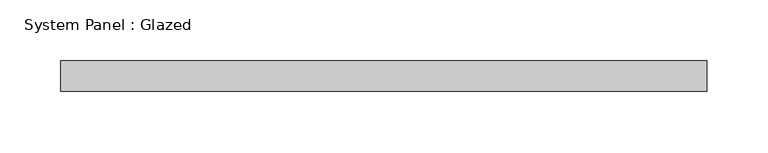
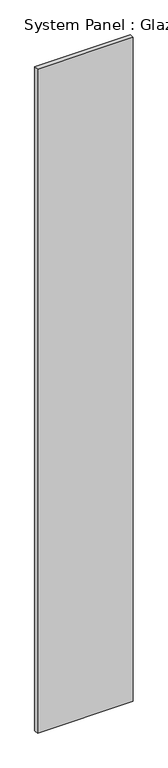
"""IFC4 building model written with IfcOpenShell, lengths in millimetres: plate geometry, System Panel : Glazed."""

from ifc_helpers import new_model, si_unit, origin, origin_with_axes, place, context, project, spatial, polyline, outline, extrude, source, transform, mapped, element, save


def system_panel_glazed_88fcc8eb(model_context):
    return source(origin(), model_context, "Body", "SweptSolid", [
        extrude(outline(polyline([(266.25, 24.5), (-266.25, 24.5), (-266.25, 49.5), (266.25, 49.5), (266.25, 24.5)])), origin_with_axes(), (0.0, 0.0, 1.0), 3900.0),
    ])


if __name__ == "__main__":
    model = new_model("IFC4")
    model_context = context("Model", 3, world=origin())
    ifc_project = project(units=[si_unit("LENGTHUNIT", "METRE", prefix="MILLI")], contexts=[model_context])
    site = spatial("IfcSite", under=ifc_project)
    building = spatial("IfcBuilding", under=site)
    placement = place(None, origin())
    system_panel_glazed_shape = system_panel_glazed_88fcc8eb(model_context)
    element("IfcPlate", 1, ObjectType="System Panel : Glazed", at=placement, inside=building, context=model_context, shape_type="MappedRepresentation", body=[
        mapped(system_panel_glazed_shape, transform((0.0, 0.0, 0.0), x_axis=(1.0, 0.0, 0.0), y_axis=(0.0, 1.0, 0.0), z_axis=(0.0, 0.0, 1.0))),
    ])
    save(model, "model.ifc")

# Revit data of these elements
# Type "System Panel : Glazed"
#   Keynote = "H11"
#   Construction Type Id = "GSP4R"
#   Analytic Construction = "1/8 in Pilkington single glazing"
#   Visual Light Transmittance = 0.9
#   Solar Heat Gain Coefficient = 0.86
#   Heat Transfer Coefficient (U) = 6.7069 W/(m²·K)
#   Define Thermal Properties by = 1
# Element 1 (IfcPlate, "System Panel : Glazed")
#   Materials on its faces: "Glass"
# Materials
#   "Glass": class "Glass", colour RGB 0 128 192, transparency 0.9, Description = "Soda Lime Glass", Cost = 0
